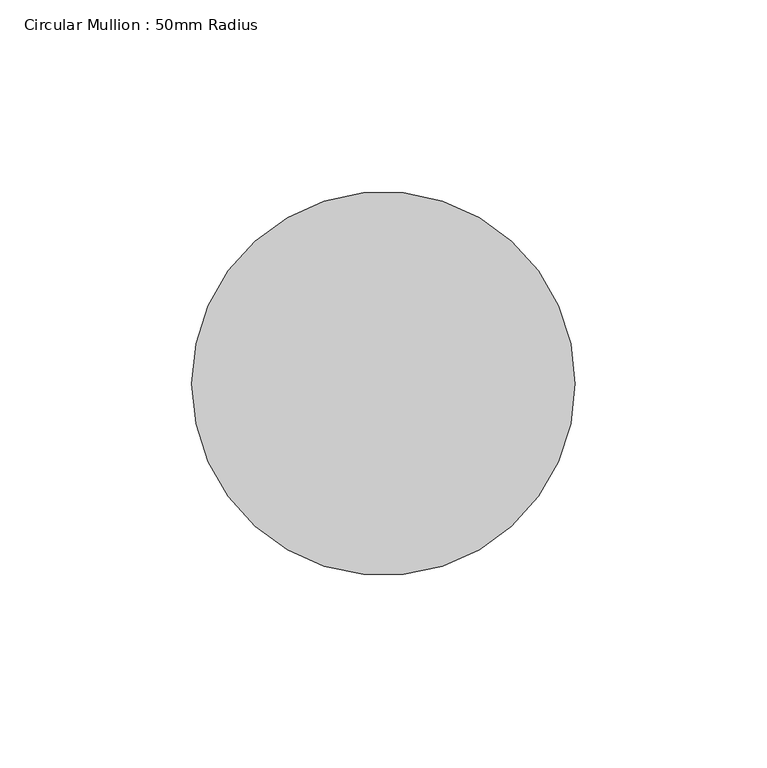
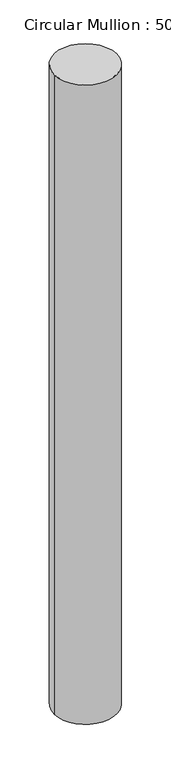
"""IFC4 building model written with IfcOpenShell, lengths in millimetres: member geometry, Circular Mullion : 50mm Radius."""

from ifc_helpers import new_model, si_unit, point, frame, origin, origin_2d, place, context, project, spatial, circle_curve, trimmed, segment, composite_curve, outline, extrude, source, transform, mapped, element, save


def circular_mullion_50mm_radius_36c1ed22(model_context):
    return source(origin(), model_context, "Body", "SweptSolid", [
        extrude(outline(composite_curve([segment(trimmed(circle_curve(origin_2d(), 50.0), [point((50.0, 0.0))], [point((-50.0, 0.0))], False, "CARTESIAN"), True, "CONTINUOUS"), segment(trimmed(circle_curve(origin_2d(), 50.0), [point((-50.0, 0.0))], [point((50.0, 0.0))], False, "CARTESIAN"), True, "CONTINUOUS")], self_intersect=False)), frame((0.0, 0.0, -1082.7457922), z_axis=(0.0, 0.0, 1.0), x_axis=(1.0, 0.0, 0.0)), (0.0, 0.0, 1.0), 1082.7457922),
    ])


if __name__ == "__main__":
    model = new_model("IFC4")
    model_context = context("Model", 3, world=origin())
    ifc_project = project(units=[si_unit("LENGTHUNIT", "METRE", prefix="MILLI")], contexts=[model_context])
    site = spatial("IfcSite", under=ifc_project)
    building = spatial("IfcBuilding", under=site)
    placement = place(None, origin())
    circular_mullion_50mm_radius_shape = circular_mullion_50mm_radius_36c1ed22(model_context)
    element("IfcMember", 1, ObjectType="Circular Mullion : 50mm Radius", at=placement, inside=building, context=model_context, shape_type="MappedRepresentation", body=[
        mapped(circular_mullion_50mm_radius_shape, transform((0.0, 0.0, 0.0), x_axis=(1.0, 0.0, 0.0), y_axis=(0.0, 1.0, 0.0), z_axis=(0.0, 0.0, 1.0))),
    ])
    save(model, "model.ifc")

# Revit data of these elements
# Type "Circular Mullion : 50mm Radius"
#   built-in parameter 1007350 = 0.164042 (stored number, unit not read)
# Element 1 (IfcMember, "Circular Mullion : 50mm Radius")
#   Materials on its faces: "Aluminium"
# Materials
#   "Aluminium": class "Metal", colour RGB 247 247 247, transparency 0, Description = "Aluminium 6061", Cost = 0
